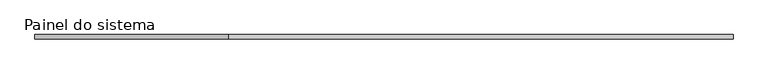
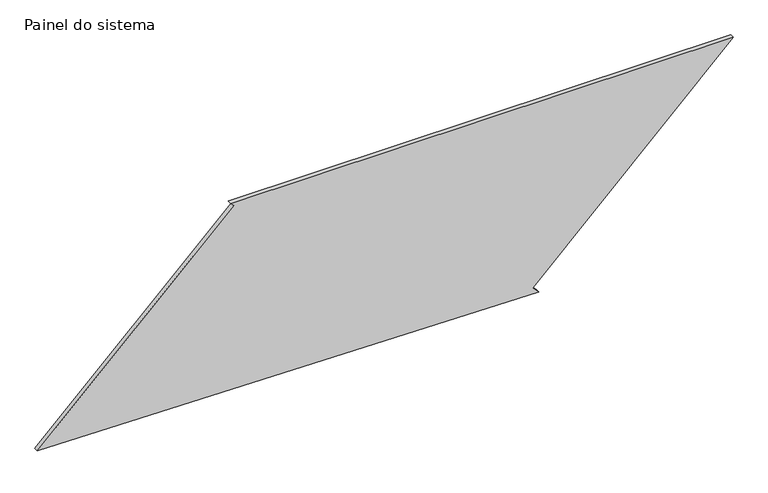
"""IFC4 building model written with IfcOpenShell, lengths in millimetres: plate geometry, Painel do sistema : Envidraçado."""

from ifc_helpers import new_model, si_unit, frame, origin, place, context, project, spatial, polyline, outline, extrude, source, transform, mapped, element, save


def painel_do_sistema_804256de(model_context):
    return source(origin(), model_context, "Body", "SweptSolid", [
        extrude(outline(polyline([(0.0, 912.2974811), (35.8123219, 877.4051094), (1198.0034185, 2070.2378009), (1198.0034185, -920.1798657), (1180.0972576, -902.7336798), (42.5840888, -2070.2378009), (0.0, 912.2974811)])), frame((0.0, 24.5, 0.0), z_axis=(0.0, 1.0, 0.0), x_axis=(0.0, 0.0, 1.0)), (0.0, 0.0, 1.0), 25.0),
    ])


if __name__ == "__main__":
    model = new_model("IFC4")
    model_context = context("Model", 3, world=origin())
    ifc_project = project(units=[si_unit("LENGTHUNIT", "METRE", prefix="MILLI")], contexts=[model_context])
    site = spatial("IfcSite", under=ifc_project)
    building = spatial("IfcBuilding", under=site)
    placement = place(None, origin())
    painel_do_sistema_shape = painel_do_sistema_804256de(model_context)
    element("IfcPlate", 1, ObjectType="Painel do sistema : Envidraçado", at=placement, inside=building, context=model_context, shape_type="MappedRepresentation", body=[
        mapped(painel_do_sistema_shape, transform((0.0, 0.0, 0.0), x_axis=(1.0, 0.0, 0.0), y_axis=(0.0, 1.0, 0.0), z_axis=(0.0, 0.0, 1.0))),
    ])
    save(model, "model.ifc")

# Revit data of these elements
# Type "Painel do sistema : Envidraçado"
#   Construction Type Id = "GSP4R"
#   Analytic Construction = "Vidraça única Pilkington 1/8 pol"
#   Visual Light Transmittance = 0.9
#   Solar Heat Gain Coefficient = 0.86
#   Heat Transfer Coefficient (U) = 6.7069 W/(m²·K)
# Element 1 (IfcPlate, "Painel do sistema : Envidraçado")
#   Materials on its faces: "Vidro"
# Materials
#   "Vidro": class "Vidro", colour RGB 0 128 192, transparency 0.9, Description = "Vidro de sílica", Cost = 0
